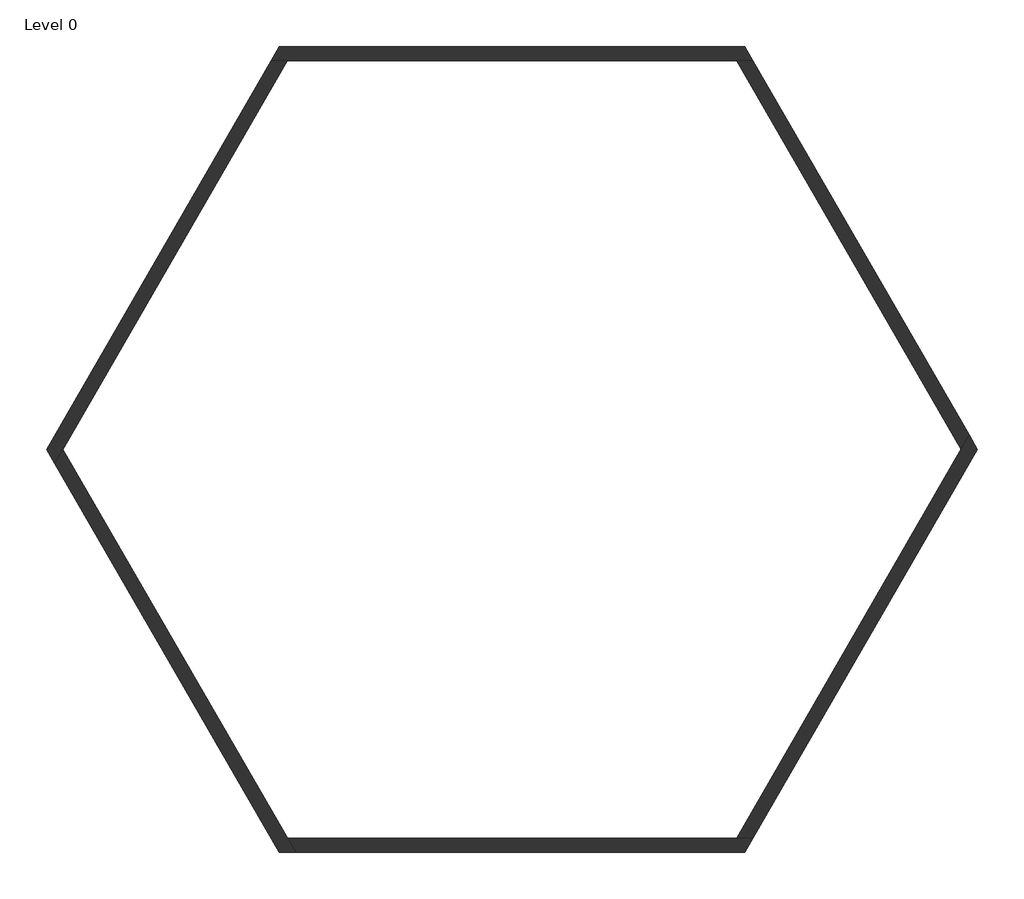
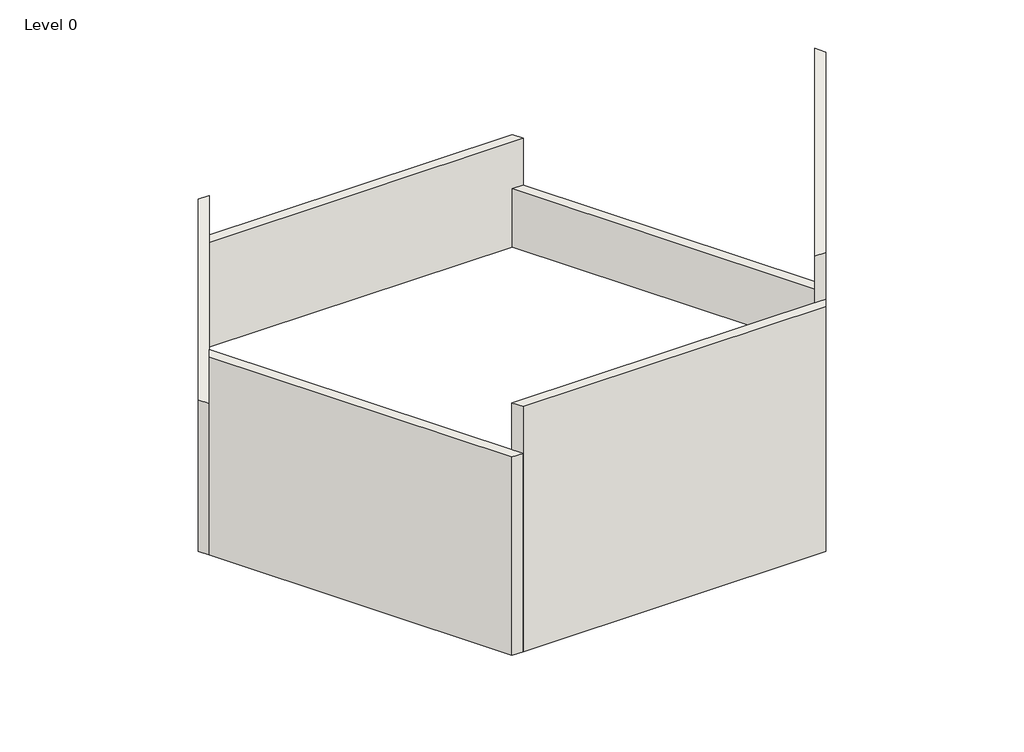
# One storey: 6 walls.
"""IFC4 building model written with IfcOpenShell, lengths in millimetres."""

from ifc_helpers import new_model, si_unit, origin, origin_with_axes, place, context, project, spatial, polyline, outline, extrude, faceted_brep, element, save

model = new_model("IFC4")

# Units and contexts
model_context = context("Model", 3, world=origin())
ifc_project = project(units=[si_unit("LENGTHUNIT", "METRE", prefix="MILLI")], contexts=[model_context])

# Site, building, storey
site = spatial("IfcSite", under=ifc_project)
building = spatial("IfcBuilding", under=site)
storey = spatial("IfcBuildingStorey", under=building, Name="Level 0", Elevation=0.0)

# Walls
placement = place(None, origin())
element("IfcWall", 1, ObjectType="Wall-Ext_102Bwk-50Air-45Ins-100DBlk-12P", at=placement, inside=storey, context=model_context, shape_type="Brep", body=[
    faceted_brep([(5089.4892917, 8815.2540378, 0.0), (-5089.4892917, 8815.2540378, 0.0), (-5089.4892917, 8815.2540378, 3600.0), (5089.4892917, 8815.2540378, 3600.0), (5268.4678752, 8505.2540378, 0.0), (5268.4678752, 8505.2540378, 2000.0), (5268.4678752, 8505.2540378, 3600.0), (-5268.4678752, 8505.2540378, 3600.0), (-5268.4678752, 8505.2540378, 0.0), (-4910.5107083, 8505.2540378, 0.0), (4910.5107083, 8505.2540378, 0.0)], [[[0, 1, 2, 3]], [[4, 5, 6, 7, 8, 9, 10]], [[1, 0, 4, 10, 9, 8]], [[3, 2, 7, 6]], [[2, 1, 8, 7]], [[0, 3, 6, 5, 4]]]),
])
element("IfcWall", 2, ObjectType="Wall-Ext_102Bwk-50Air-45Ins-100DBlk-12P", at=placement, inside=storey, context=model_context, shape_type="Brep", body=[
    faceted_brep([(-5268.4678752, 8505.2540378, 0.0), (-10178.9785834, 0.0, 0.0), (-10178.9785834, 0.0, 5200.0), (-5268.4678752, 8505.2540378, 5200.0), (-5268.4678752, 8505.2540378, 3600.0), (-4910.5107083, 8505.2540378, 0.0), (-4910.5107083, 8505.2540378, 5200.0), (-10000.0, -310.0, 5200.0), (-10000.0, -310.0, 0.0), (-9821.0214166, 0.0, 0.0)], [[[0, 1, 2, 3, 4]], [[5, 6, 7, 8, 9]], [[1, 0, 5, 9, 8]], [[3, 2, 7, 6]], [[2, 1, 8, 7]], [[0, 4, 3, 6, 5]]]),
])
element("IfcWall", 3, ObjectType="Wall-Ext_102Bwk-50Air-45Ins-100DBlk-12P", at=placement, inside=storey, context=model_context, shape_type="Brep", body=[
    faceted_brep([(-10000.0, -310.0, 0.0), (-5089.4892917, -8815.2540378, 0.0), (-5089.4892917, -8815.2540378, 6800.0), (-10000.0, -310.0, 6800.0), (-10000.0, -310.0, 5200.0), (-9821.0214166, 0.0, 0.0), (-9821.0214166, 0.0, 6800.0), (-4731.5321248, -8815.2540378, 6800.0), (-4731.5321248, -8815.2540378, 0.0), (-4910.5107083, -8505.2540378, 0.0)], [[[0, 1, 2, 3, 4]], [[5, 6, 7, 8, 9]], [[1, 0, 5, 9, 8]], [[3, 2, 7, 6]], [[2, 1, 8, 7]], [[0, 4, 3, 6, 5]]]),
])
element("IfcWall", 4, ObjectType="Wall-Ext_102Bwk-50Air-45Ins-100DBlk-12P", at=placement, inside=storey, context=model_context, shape_type="Brep", body=[
    faceted_brep([(-4731.5321248, -8815.2540378, 0.0), (5089.4892917, -8815.2540378, 0.0), (5089.4892917, -8815.2540378, 8400.0), (-4731.5321248, -8815.2540378, 8400.0), (-4731.5321248, -8815.2540378, 6800.0), (-4910.5107083, -8505.2540378, 0.0), (-4910.5107083, -8505.2540378, 8400.0), (5268.4678752, -8505.2540378, 8400.0), (5268.4678752, -8505.2540378, 0.0), (4910.5107083, -8505.2540378, 0.0)], [[[0, 1, 2, 3, 4]], [[5, 6, 7, 8, 9]], [[1, 0, 5, 9, 8]], [[3, 2, 7, 6]], [[2, 1, 8, 7]], [[0, 4, 3, 6, 5]]]),
])
element("IfcWall", 5, ObjectType="Wall-Ext_102Bwk-50Air-45Ins-100DBlk-12P", at=placement, inside=storey, context=model_context, shape_type="Brep", body=[
    faceted_brep([(5268.4678752, -8505.2540378, 0.0), (10178.9785834, 0.0, 0.0), (10178.9785834, 0.0, 10000.0), (5268.4678752, -8505.2540378, 10000.0), (5268.4678752, -8505.2540378, 8400.0), (4910.5107083, -8505.2540378, 0.0), (4910.5107083, -8505.2540378, 10000.0), (10000.0, 310.0, 10000.0), (10000.0, 310.0, 2000.0), (10000.0, 310.0, 0.0), (9821.0214166, 0.0, 0.0)], [[[0, 1, 2, 3, 4]], [[5, 6, 7, 8, 9, 10]], [[1, 0, 5, 10, 9]], [[3, 2, 7, 6]], [[0, 4, 3, 6, 5]], [[2, 1, 9, 8, 7]]]),
])
element("IfcWall", 6, ObjectType="Wall-Ext_102Bwk-50Air-45Ins-100DBlk-12P", at=placement, inside=storey, context=model_context, shape_type="SweptSolid", body=[
    extrude(outline(polyline([(5268.4678752, 8505.2540378), (10000.0, 310.0), (9821.0214166, 0.0), (4910.5107083, 8505.2540378), (5268.4678752, 8505.2540378)])), origin_with_axes(), (0.0, 0.0, 1.0), 2000.0),
])

save(model, "model.ifc")

# Revit data of these elements
# Project information
#   Project Issue Date = "Issue Date"
#   Project Status = "Project Status"
#   Client Name = "Owner"
#   Project Address = "Enter address here"
#   Project Name = "Project Name"
#   Project Number = "Project Number"
# Type "Wall-Ext_102Bwk-50Air-45Ins-100DBlk-12P"
#   Keynote = "F10"
#   Layers, outside or top first: 102.5 mm "Brick, Common" (function 4); 50 mm "Air" (function 3); 45 mm "Fiberglass Batt" (function 3); 100 mm "Concrete Masonry Units _High Density" (function 1); 12.5 mm "Plaster" (function 5)
# Element 1 (IfcWall, "Wall-Ext_102Bwk-50Air-45Ins-100DBlk-12P")
#   Top Offset = 0 mm
#   Base Offset = 0 mm
#   Unconnected Height = 3600 mm
#   wall height = 3600 mm
#   Phase Created = New Construction
#   Base Constraint = Level 0
#   Materials on its faces: "Plaster", "Default Wall", "Brick, Common"
# Element 2 (IfcWall, "Wall-Ext_102Bwk-50Air-45Ins-100DBlk-12P")
#   Top Offset = 0 mm
#   Base Offset = 0 mm
#   Unconnected Height = 5200 mm
#   wall height = 5200 mm
#   Phase Created = New Construction
#   Base Constraint = Level 0
#   Materials on its faces: "Default Wall", "Plaster", "Brick, Common"
# Element 3 (IfcWall, "Wall-Ext_102Bwk-50Air-45Ins-100DBlk-12P")
#   Top Offset = 0 mm
#   Base Offset = 0 mm
#   Unconnected Height = 6800 mm
#   wall height = 6800 mm
#   Phase Created = New Construction
#   Base Constraint = Level 0
#   Materials on its faces: "Default Wall", "Plaster", "Brick, Common"
# Element 4 (IfcWall, "Wall-Ext_102Bwk-50Air-45Ins-100DBlk-12P")
#   Top Offset = 0 mm
#   Base Offset = 0 mm
#   Unconnected Height = 8400 mm
#   wall height = 8400 mm
#   Phase Created = New Construction
#   Base Constraint = Level 0
#   Materials on its faces: "Default Wall", "Plaster", "Brick, Common"
# Element 5 (IfcWall, "Wall-Ext_102Bwk-50Air-45Ins-100DBlk-12P")
#   Top Offset = 0 mm
#   Base Offset = 0 mm
#   Unconnected Height = 10000 mm
#   wall height = 10000 mm
#   Phase Created = New Construction
#   Base Constraint = Level 0
#   Materials on its faces: "Default Wall", "Plaster", "Brick, Common"
# Element 6 (IfcWall, "Wall-Ext_102Bwk-50Air-45Ins-100DBlk-12P")
#   Top Offset = 0 mm
#   Base Offset = 0 mm
#   Unconnected Height = 2000 mm
#   wall height = 2000 mm
#   Phase Created = New Construction
#   Base Constraint = Level 0
#   Materials on its faces: "Default Wall", "Plaster", "Brick, Common"
# Materials
#   "Brick, Common": class "Masonry", colour RGB 170 100 105, transparency 0, Description = "Common brick", Cost = 0
#   "Air": class "Gas", colour RGB 255 255 255, transparency 0, Description = "Air", Cost = 0
#   "Fiberglass Batt": class "Generic", colour RGB 127 127 127, transparency 0, Description = "Fiberglass batt insulation", Cost = 0
#   "Concrete Masonry Units _High Density": class "Masonry", colour RGB 181 181 181, transparency 0, Description = "Concrete masonry units", Cost = 0
#   "Plaster": class "Generic", colour RGB 249 249 249, transparency 0, Description = "Plaster", Cost = 0
#   "Default Wall": class "Miscellaneous", colour RGB 128 128 128, transparency 0, Comments = "Rendering appearance not upgraded ", Cost = 0
